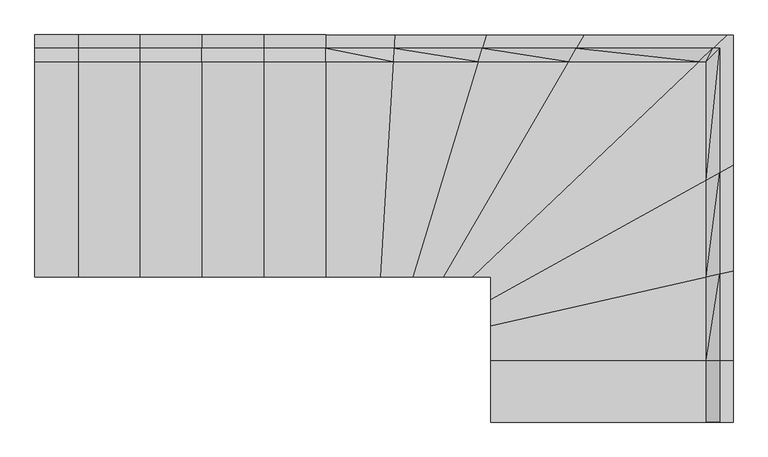
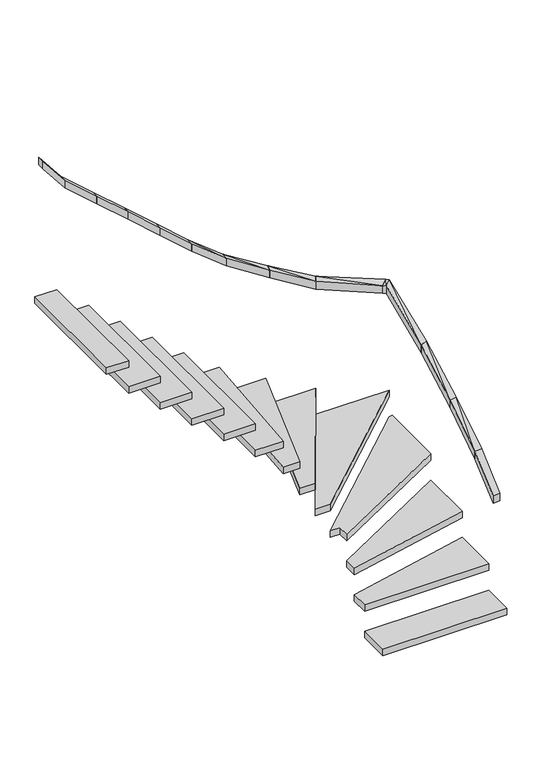
"""IFC4 building model written with IfcOpenShell, lengths in millimetres: stair geometry, 0_3d."""

from ifc_helpers import new_model, si_unit, frame, origin, origin_with_axes, place, context, project, spatial, polyline, outline, extrude, faceted_brep, source, transform, mapped, element, save


def stair_fc5a61e0(model_context):
    return source(origin(), model_context, "Body", "SolidModel", [
        faceted_brep([(1662.1084245, 1390.0, 2104.8571429), (2010.4511549, 1390.0, 1902.7142857), (1981.4161719, 1340.0, 1902.7142857), (1646.8946419, 1340.0, 2104.8571429), (1981.4161719, 1340.0, 1960.7142857), (2010.4511549, 1390.0, 1960.7142857), (1662.1084245, 1390.0, 2162.8571429), (1646.8946419, 1340.0, 2162.8571429)], [[[0, 1, 2]], [[3, 0, 2]], [[4, 5, 6]], [[7, 4, 6]], [[4, 2, 1, 5]], [[5, 1, 0, 6]], [[6, 0, 3, 7]], [[7, 3, 2, 4]]]),
        faceted_brep([(2545.0, 1390.0, 1690.0645825), (2545.0, 928.5523018, 1498.4285714), (2495.0, 900.8094062, 1498.4285714), (2495.0, 1340.0, 1688.4852367), (2519.7001625, 1390.0, 1700.5714286), (2467.0707412, 1340.0, 1700.5714286), (2495.0, 900.8094062, 1556.4285714), (2545.0, 928.5523018, 1556.4285714), (2545.0, 1390.0, 1748.0645825), (2495.0, 1340.0, 1746.4852367), (2519.7001625, 1390.0, 1758.5714286), (2467.0707412, 1340.0, 1758.5714286)], [[[0, 1, 2]], [[3, 0, 2]], [[4, 0, 3]], [[5, 4, 3]], [[6, 7, 8]], [[9, 6, 8]], [[9, 8, 10]], [[11, 9, 10]], [[6, 2, 1, 7]], [[7, 1, 0, 8]], [[8, 0, 4, 10]], [[10, 4, 5, 11]], [[11, 5, 3, 9]], [[9, 3, 2, 6]]]),
        extrude(outline(polyline([(1625.0, 540.0), (1516.8564445, 540.0), (2039.4861379, 1440.0), (2572.3295839, 1440.0), (1625.0, 540.0)])), frame((0.0, 0.0, 808.5714286), z_axis=(0.0, 0.0, 1.0), x_axis=(1.0, 0.0, 0.0)), (0.0, 0.0, 1.0), 50.0),
        faceted_brep([(2545.0, 551.5263914, 1296.2857143), (2545.0, 230.0, 1094.1428571), (2495.0, 230.0, 1094.1428571), (2495.0, 540.0855925, 1296.2857143), (2495.0, 230.0, 1152.1428571), (2545.0, 230.0, 1152.1428571), (2545.0, 551.5263914, 1354.2857143), (2495.0, 540.0855925, 1354.2857143)], [[[0, 1, 2]], [[3, 0, 2]], [[4, 5, 6]], [[7, 4, 6]], [[4, 2, 1, 5]], [[5, 1, 0, 6]], [[6, 0, 3, 7]], [[7, 3, 2, 4]]]),
        extrude(outline(polyline([(1403.4741197, 540.0), (1283.1567001, 540.0), (1337.6396267, 1440.0), (1677.3222071, 1440.0), (1403.4741197, 540.0)])), frame((0.0, 0.0, 1212.8571429), z_axis=(0.0, 0.0, 1.0), x_axis=(1.0, 0.0, 0.0)), (0.0, 0.0, 1.0), 50.0),
        extrude(outline(polyline([(2971.4285714, 620.3981634), (2913.4285714, 620.3981634), (2711.2857143, 850.3981634), (2769.2857143, 850.3981634), (2971.4285714, 620.3981634)])), frame((0.0, 1340.0, 0.0), z_axis=(0.0, 1.0, 0.0), x_axis=(0.0, 0.0, 1.0)), (0.0, 0.0, 1.0), 50.0),
        faceted_brep([(2545.0, 928.5523018, 1498.4285714), (2545.0, 551.5263914, 1296.2857143), (2495.0, 540.0855925, 1296.2857143), (2495.0, 900.8094062, 1498.4285714), (2495.0, 540.0855925, 1354.2857143), (2545.0, 551.5263914, 1354.2857143), (2545.0, 928.5523018, 1556.4285714), (2495.0, 900.8094062, 1556.4285714)], [[[0, 1, 2]], [[3, 0, 2]], [[4, 5, 6]], [[7, 4, 6]], [[4, 2, 1, 5]], [[5, 1, 0, 6]], [[6, 0, 3, 7]], [[7, 3, 2, 4]]]),
        faceted_brep([(1080.3981634, 1390.0, 2509.1428571), (1334.6127974, 1390.0, 2307.0), (1331.5859682, 1340.0, 2307.0), (1080.3981634, 1340.0, 2509.1428571), (1331.5859682, 1340.0, 2365.0), (1334.6127974, 1390.0, 2365.0), (1080.3981634, 1390.0, 2567.1428571), (1080.3981634, 1340.0, 2567.1428571)], [[[0, 1, 2]], [[3, 0, 2]], [[4, 5, 6]], [[7, 4, 6]], [[4, 2, 1, 5]], [[5, 1, 0, 6]], [[6, 0, 3, 7]], [[7, 3, 2, 4]]]),
        extrude(outline(polyline([(160.3981634, 540.0), (0.0, 540.0), (0.0, 1440.0), (160.3981634, 1440.0), (160.3981634, 540.0)])), frame((0.0, 0.0, 2425.7142857), z_axis=(0.0, 0.0, 1.0), x_axis=(1.0, 0.0, 0.0)), (0.0, 0.0, 1.0), 50.0),
        faceted_brep([(1334.6127974, 1390.0, 2307.0), (1662.1084245, 1390.0, 2104.8571429), (1646.8946419, 1340.0, 2104.8571429), (1331.5859682, 1340.0, 2307.0), (1646.8946419, 1340.0, 2162.8571429), (1662.1084245, 1390.0, 2162.8571429), (1334.6127974, 1390.0, 2365.0), (1331.5859682, 1340.0, 2365.0)], [[[0, 1, 2]], [[3, 0, 2]], [[4, 5, 6]], [[7, 4, 6]], [[4, 2, 1, 5]], [[5, 1, 0, 6]], [[6, 0, 3, 7]], [[7, 3, 2, 4]]]),
        extrude(outline(polyline([(620.3981634, 540.0), (390.3981634, 540.0), (390.3981634, 1440.0), (620.3981634, 1440.0), (620.3981634, 540.0)])), frame((0.0, 0.0, 2021.4285714), z_axis=(0.0, 0.0, 1.0), x_axis=(1.0, 0.0, 0.0)), (0.0, 0.0, 1.0), 50.0),
        extrude(outline(polyline([(1080.3981634, 540.0), (850.3981634, 540.0), (850.3981634, 1440.0), (1080.3981634, 1440.0), (1080.3981634, 540.0)])), frame((0.0, 0.0, 1617.1428571), z_axis=(0.0, 0.0, 1.0), x_axis=(1.0, 0.0, 0.0)), (0.0, 0.0, 1.0), 50.0),
        extrude(outline(polyline([(390.3981634, 540.0), (160.3981634, 540.0), (160.3981634, 1440.0), (390.3981634, 1440.0), (390.3981634, 540.0)])), frame((0.0, 0.0, 2223.5714286), z_axis=(0.0, 0.0, 1.0), x_axis=(1.0, 0.0, 0.0)), (0.0, 0.0, 1.0), 50.0),
        extrude(outline(polyline([(1516.8564445, 540.0), (1403.4741197, 540.0), (1677.3222071, 1440.0), (2039.4861379, 1440.0), (1516.8564445, 540.0)])), frame((0.0, 0.0, 1010.7142857), z_axis=(0.0, 0.0, 1.0), x_axis=(1.0, 0.0, 0.0)), (0.0, 0.0, 1.0), 50.0),
        extrude(outline(polyline([(3577.8571429, 0.0), (3519.8571429, 0.0), (3317.7142857, 160.3981634), (3375.7142857, 160.3981634), (3577.8571429, 0.0)])), frame((0.0, 1340.0, 0.0), z_axis=(0.0, 1.0, 0.0), x_axis=(0.0, 0.0, 1.0)), (0.0, 0.0, 1.0), 50.0),
        extrude(outline(polyline([(1695.0, 230.0), (1695.0, 357.0328096), (2595.0, 562.9671904), (2595.0, 230.0), (1695.0, 230.0)])), frame((0.0, 0.0, 202.1428571), z_axis=(0.0, 0.0, 1.0), x_axis=(1.0, 0.0, 0.0)), (0.0, 0.0, 1.0), 50.0),
        extrude(outline(polyline([(1695.0, 357.0328096), (1695.0, 456.9230769), (2595.0, 956.2951974), (2595.0, 562.9671904), (1695.0, 357.0328096)])), frame((0.0, 0.0, 404.2857143), z_axis=(0.0, 0.0, 1.0), x_axis=(1.0, 0.0, 0.0)), (0.0, 0.0, 1.0), 50.0),
        extrude(outline(polyline([(1695.0, 0.0), (1695.0, 230.0), (2595.0, 230.0), (2595.0, 0.0), (1695.0, 0.0)])), origin_with_axes(), (0.0, 0.0, 1.0), 50.0),
        faceted_brep([(2010.4511549, 1390.0, 1902.7142857), (2519.7001625, 1390.0, 1700.5714286), (2467.0707412, 1340.0, 1700.5714286), (1981.4161719, 1340.0, 1902.7142857), (2467.0707412, 1340.0, 1758.5714286), (2519.7001625, 1390.0, 1758.5714286), (2010.4511549, 1390.0, 1960.7142857), (1981.4161719, 1340.0, 1960.7142857)], [[[0, 1, 2]], [[3, 0, 2]], [[4, 5, 6]], [[7, 4, 6]], [[4, 2, 1, 5]], [[5, 1, 0, 6]], [[6, 0, 3, 7]], [[7, 3, 2, 4]]]),
        extrude(outline(polyline([(2769.2857143, 850.3981634), (2711.2857143, 850.3981634), (2509.1428571, 1080.3981634), (2567.1428571, 1080.3981634), (2769.2857143, 850.3981634)])), frame((0.0, 1340.0, 0.0), z_axis=(0.0, 1.0, 0.0), x_axis=(0.0, 0.0, 1.0)), (0.0, 0.0, 1.0), 50.0),
        extrude(outline(polyline([(230.0, 1152.1428571), (230.0, 1094.1428571), (0.0, 892.0), (0.0, 950.0), (230.0, 1152.1428571)])), frame((2495.0, 0.0, 0.0), z_axis=(1.0, 0.0, 0.0), x_axis=(0.0, 1.0, 0.0)), (0.0, 0.0, 1.0), 50.0),
        extrude(outline(polyline([(3375.7142857, 160.3981634), (3317.7142857, 160.3981634), (3115.5714286, 390.3981634), (3173.5714286, 390.3981634), (3375.7142857, 160.3981634)])), frame((0.0, 1340.0, 0.0), z_axis=(0.0, 1.0, 0.0), x_axis=(0.0, 0.0, 1.0)), (0.0, 0.0, 1.0), 50.0),
        extrude(outline(polyline([(3173.5714286, 390.3981634), (3115.5714286, 390.3981634), (2913.4285714, 620.3981634), (2971.4285714, 620.3981634), (3173.5714286, 390.3981634)])), frame((0.0, 1340.0, 0.0), z_axis=(0.0, 1.0, 0.0), x_axis=(0.0, 0.0, 1.0)), (0.0, 0.0, 1.0), 50.0),
        extrude(outline(polyline([(1695.0, 456.9230769), (1695.0, 540.0), (1625.0, 540.0), (2572.3295839, 1440.0), (2595.0, 1440.0), (2595.0, 956.2951974), (1695.0, 456.9230769)])), frame((0.0, 0.0, 606.4285714), z_axis=(0.0, 0.0, 1.0), x_axis=(1.0, 0.0, 0.0)), (0.0, 0.0, 1.0), 50.0),
        extrude(outline(polyline([(850.3981634, 540.0), (620.3981634, 540.0), (620.3981634, 1440.0), (850.3981634, 1440.0), (850.3981634, 540.0)])), frame((0.0, 0.0, 1819.2857143), z_axis=(0.0, 0.0, 1.0), x_axis=(1.0, 0.0, 0.0)), (0.0, 0.0, 1.0), 50.0),
        extrude(outline(polyline([(1283.1567001, 540.0), (1080.3981634, 540.0), (1080.3981634, 1440.0), (1337.6396267, 1440.0), (1283.1567001, 540.0)])), frame((0.0, 0.0, 1415.0), z_axis=(0.0, 0.0, 1.0), x_axis=(1.0, 0.0, 0.0)), (0.0, 0.0, 1.0), 50.0),
    ])


if __name__ == "__main__":
    model = new_model("IFC4")
    model_context = context("Model", 3, world=origin())
    ifc_project = project(units=[si_unit("LENGTHUNIT", "METRE", prefix="MILLI")], contexts=[model_context])
    site = spatial("IfcSite", under=ifc_project)
    building = spatial("IfcBuilding", under=site)
    placement = place(None, origin())
    stair_shape = stair_fc5a61e0(model_context)
    element("IfcStair", 1, ObjectType="0_3d", at=placement, inside=building, context=model_context, shape_type="MappedRepresentation", body=[
        mapped(stair_shape, transform((0.0, 0.0, 0.0), x_axis=(1.0, 0.0, 0.0), y_axis=(0.0, 1.0, 0.0), z_axis=(0.0, 0.0, 1.0))),
    ])
    save(model, "model.ifc")

# Revit data of these elements
# Element 1 (IfcStair, "0_3d")
#   Materials on its faces: "*1", "weiss"
# Materials
#   "*1": class "Unassigned", colour RGB 175 175 175, transparency 0
#   "weiss": class "Unassigned", colour RGB 255 255 255, transparency 0
